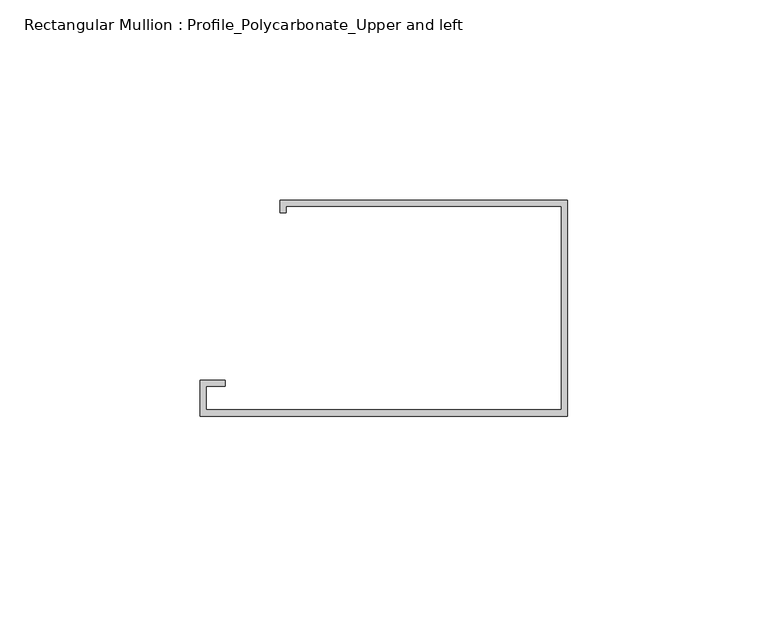
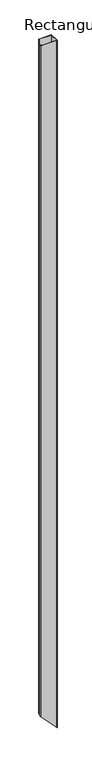
"""IFC4 building model written with IfcOpenShell, lengths in millimetres: member geometry, Rectangular Mullion : Profile_Polycarbonate_Upper and left."""

from ifc_helpers import new_model, si_unit, origin, place, context, project, spatial, faceted_brep, source, transform, mapped, element, save


def rectangular_mullion_profile_polycarbonate_upper_and_left_5b0ad0f7(model_context):
    return source(origin(), model_context, "Body", "Brep", [
        faceted_brep([(0.0, -28.984575, 0.0), (0.0, 25.015825, 0.0), (-71.9836, 25.015825, 0.0), (-71.9836, 21.840825, 0.0), (-70.3961, 21.840825, 0.0), (-70.3961, 23.428325, 0.0), (-1.5875, 23.428325, 0.0), (-1.5875, -27.397075, 0.0), (-90.4113, -27.397075, 0.0), (-90.4113, -21.580475, 0.0), (-85.6488, -21.580475, 0.0), (-85.6488, -19.992975, 0.0), (-91.9988, -19.992975, 0.0), (-91.9988, -28.984575, 0.0), (0.0, -28.984575, -4039.5062498), (0.0, 25.015825, -4039.5062498), (-71.9836, 25.015825, -3964.4608744), (-71.9836, 21.840825, -3964.4608744), (-70.3961, 21.840825, -3966.1158977), (-70.3961, 23.428325, -3966.1158977), (-1.5875, 23.428325, -4037.8512265), (-1.5875, -27.397075, -4037.8512265), (-90.4113, -27.397075, -3945.2493643), (-90.4113, -21.580475, -3945.2493643), (-85.6488, -21.580475, -3950.2144341), (-85.6488, -19.992975, -3950.2144341), (-91.9988, -19.992975, -3943.594341), (-91.9988, -28.984575, -3943.594341)], [[[0, 1, 2, 3, 4, 5, 6, 7, 8, 9, 10, 11, 12, 13]], [[1, 0, 14, 15]], [[2, 1, 15, 16]], [[3, 2, 16, 17]], [[4, 3, 17, 18]], [[5, 4, 18, 19]], [[6, 5, 19, 20]], [[7, 6, 20, 21]], [[8, 7, 21, 22]], [[9, 8, 22, 23]], [[10, 9, 23, 24]], [[11, 10, 24, 25]], [[12, 11, 25, 26]], [[13, 12, 26, 27]], [[0, 13, 27, 14]], [[14, 27, 26, 25, 24, 23, 22, 21, 20, 19, 18, 17, 16, 15]]]),
    ])


if __name__ == "__main__":
    model = new_model("IFC4")
    model_context = context("Model", 3, world=origin())
    ifc_project = project(units=[si_unit("LENGTHUNIT", "METRE", prefix="MILLI")], contexts=[model_context])
    site = spatial("IfcSite", under=ifc_project)
    building = spatial("IfcBuilding", under=site)
    placement = place(None, origin())
    rectangular_mullion_profile_polycarbonate_upper_and_left_shape = rectangular_mullion_profile_polycarbonate_upper_and_left_5b0ad0f7(model_context)
    element("IfcMember", 1, ObjectType="Rectangular Mullion : Profile_Polycarbonate_Upper and left", at=placement, inside=building, context=model_context, shape_type="MappedRepresentation", body=[
        mapped(rectangular_mullion_profile_polycarbonate_upper_and_left_shape, transform((0.0, 0.0, 0.0), x_axis=(1.0, 0.0, 0.0), y_axis=(0.0, 1.0, 0.0), z_axis=(0.0, 0.0, 1.0))),
    ])
    save(model, "model.ifc")

# Revit data of these elements
# Type "Rectangular Mullion : Profile_Polycarbonate_Upper and left"
#   built-in parameter 1007322 = 0.177167 (stored number, unit not read)
#   built-in parameter 1007321 = 0.00520833 (stored number, unit not read)
#   built-in parameter 1007320 = 0 (stored number, unit not read)
